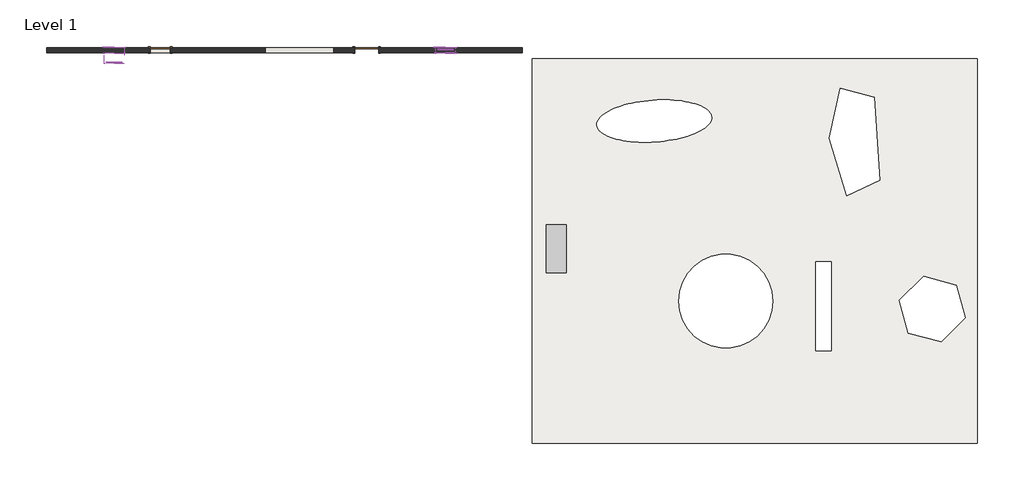
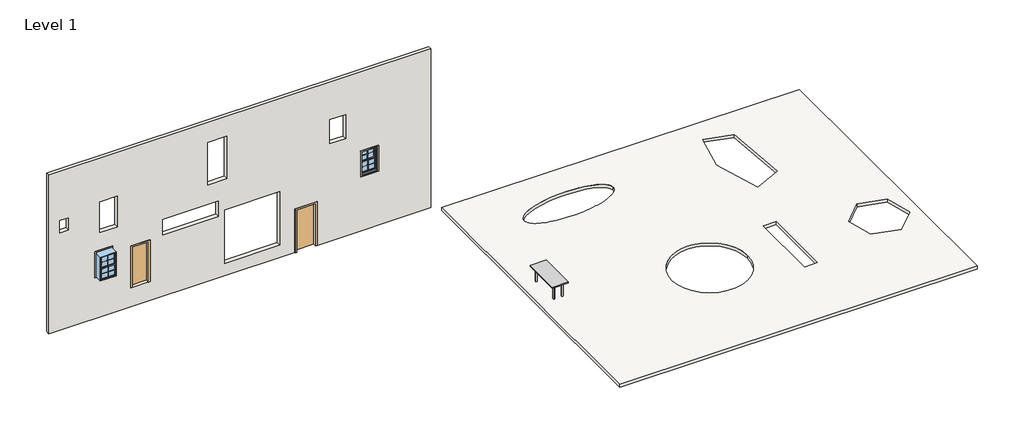
# One storey: 8 proxies, 2 doors, 2 windows, 1 furniture element, 1 slab, 1 wall.
"""IFC4 building model written with IfcOpenShell, lengths in millimetres."""

import ifcopenshell
import ifcopenshell.guid

model = None  # the IFC model being written
_history = None  # IfcOwnerHistory: only IFC2X3 demands one
_inside = {}  # id of a spatial element -> (the spatial element, [elements in it])
_under = {}  # id of a project, library or spatial element -> (it, [spatial elements below it])
_declared = {}  # id of a project -> (the project, [libraries it declares])
_typed = {}  # id of a type object -> (the type object, [elements of that type])
_made_of = {}  # id of a material, layer set ... -> (it, [elements and type objects made of it])


def new_model(schema):
    """Start an empty IFC model of exactly this schema.

    Asked for "IFC4X3", IfcOpenShell would pick the latest addendum, in which some entities
    have other attributes; the version numbers below select the first issue.
    IFC2X3 requires an IfcOwnerHistory on every rooted entity: one is made here for all.
    """
    global model, _history
    if schema == "IFC4X3":
        model = ifcopenshell.file(schema_version=(4, 3, 0, 0))
    else:
        model = ifcopenshell.file(schema=schema)
    _inside.clear()
    _under.clear()
    _declared.clear()
    _typed.clear()
    _made_of.clear()
    _history = None
    if model.schema == "IFC2X3":
        org = make("IfcOrganization", Name="unknown")
        user = make(
            "IfcPersonAndOrganization",
            ThePerson=make("IfcPerson", FamilyName="unknown"),
            TheOrganization=org,
        )
        app = make(
            "IfcApplication",
            ApplicationDeveloper=org,
            Version="unknown",
            ApplicationFullName="unknown",
            ApplicationIdentifier="unknown",
        )
        _history = make(
            "IfcOwnerHistory",
            OwningUser=user,
            OwningApplication=app,
            ChangeAction="ADDED",
            CreationDate=0,
        )
    return model


def make(cls, **values):
    """One entity of the class cls with the attributes given. An attribute that is None is left unset."""
    return model.create_entity(
        cls, **{name: value for name, value in values.items() if value is not None}
    )


def rooted(cls, **values):
    """An entity with a GlobalId (a new one), such as an element, a storey or a relation."""
    return make(cls, GlobalId=ifcopenshell.guid.new(), OwnerHistory=_history, **values)


def si_unit(unit_type, name, prefix=None):
    """IfcSIUnit, for example si_unit("LENGTHUNIT", "METRE", prefix="MILLI")."""
    return make("IfcSIUnit", UnitType=unit_type, Prefix=prefix, Name=name)


def assignment(units):
    """IfcUnitAssignment: the units of a project."""
    return None if units is None else make("IfcUnitAssignment", Units=units)


def point(xyz):
    """IfcCartesianPoint."""
    return None if xyz is None else make("IfcCartesianPoint", Coordinates=xyz)


def direction(xyz):
    """IfcDirection."""
    return None if xyz is None else make("IfcDirection", DirectionRatios=xyz)


def frame(location, z_axis=None, x_axis=None):
    """IfcAxis2Placement3D, a coordinate frame: its origin and axes. An axis left out is left unset."""
    return make(
        "IfcAxis2Placement3D",
        Location=point(location),
        Axis=direction(z_axis),
        RefDirection=direction(x_axis),
    )


def origin():
    """The frame at (0, 0, 0) with its axes left unset."""
    return frame((0.0, 0.0, 0.0))


def origin_with_axes():
    """The frame at (0, 0, 0) with the z axis (0, 0, 1) and the x axis (1, 0, 0) written out."""
    return frame((0.0, 0.0, 0.0), z_axis=(0.0, 0.0, 1.0), x_axis=(1.0, 0.0, 0.0))


def place(relative_to, where):
    """IfcLocalPlacement: puts the frame where relative to a parent placement (None: the world)."""
    return make(
        "IfcLocalPlacement", PlacementRelTo=relative_to, RelativePlacement=where
    )


def context(
    kind, dimensions, precision=None, world=None, true_north=None, identifier=None
):
    """IfcGeometricRepresentationContext, for example the 3D "Model" context."""
    return make(
        "IfcGeometricRepresentationContext",
        ContextIdentifier=identifier,
        ContextType=kind,
        CoordinateSpaceDimension=dimensions,
        Precision=precision,
        WorldCoordinateSystem=world,
        TrueNorth=true_north,
    )


def project(units=None, contexts=None):
    """IfcProject with its units and contexts."""
    return rooted(
        "IfcProject",
        Name="project",
        RepresentationContexts=contexts,
        UnitsInContext=assignment(units),
    )


def spatial(cls, under=None, at=None, **own):
    """A site, building, storey or space (cls), placed at a placement, below another one or the project."""
    s = rooted(cls, ObjectPlacement=at, **own)
    if under is not None:
        _under.setdefault(under.id(), (under, []))[1].append(s)
    return s


def polyline(points):
    """IfcPolyline through the points."""
    return make("IfcPolyline", Points=[point(p) for p in points])


def circle_curve(where, radius):
    """IfcCircle in the frame where."""
    return make("IfcCircle", Position=where, Radius=radius)


def ellipse_curve(where, semi_axis1, semi_axis2):
    """IfcEllipse in the frame where."""
    return make(
        "IfcEllipse", Position=where, SemiAxis1=semi_axis1, SemiAxis2=semi_axis2
    )


def trimmed(basis, trim1, trim2, sense, master):
    """IfcTrimmedCurve: the piece of a basis curve between two trims."""
    return make(
        "IfcTrimmedCurve",
        BasisCurve=basis,
        Trim1=trim1,
        Trim2=trim2,
        SenseAgreement=sense,
        MasterRepresentation=master,
    )


def outline(outer, holes=None, kind="AREA"):
    """IfcArbitraryClosedProfileDef: a profile drawn as a closed curve; with holes, ...WithVoids."""
    if holes is None:
        return make("IfcArbitraryClosedProfileDef", ProfileType=kind, OuterCurve=outer)
    return make(
        "IfcArbitraryProfileDefWithVoids",
        ProfileType=kind,
        OuterCurve=outer,
        InnerCurves=holes,
    )


def extrude(swept, where, along, depth):
    """IfcExtrudedAreaSolid: the profile swept, set in the frame where, extruded along a direction by depth."""
    return make(
        "IfcExtrudedAreaSolid",
        SweptArea=swept,
        Position=where,
        ExtrudedDirection=direction(along),
        Depth=depth,
    )


def shape(context_of_items, identifier, shape_type, items):
    """IfcShapeRepresentation: the items that make up one representation, for example the "Body"."""
    return make(
        "IfcShapeRepresentation",
        ContextOfItems=context_of_items,
        RepresentationIdentifier=identifier,
        RepresentationType=shape_type,
        Items=items,
    )


def source(mapping_origin, context_of_items, identifier, shape_type, items):
    """IfcRepresentationMap: a shape defined once, which mapped items show again and again."""
    return make(
        "IfcRepresentationMap",
        MappingOrigin=mapping_origin,
        MappedRepresentation=shape(context_of_items, identifier, shape_type, items),
    )


def transform(
    local_origin,
    x_axis=None,
    y_axis=None,
    z_axis=None,
    scale=None,
    scale2=None,
    scale3=None,
    uniform=True,
):
    """IfcCartesianTransformationOperator3D, or its non-uniform kind. x_axis, y_axis, z_axis: its Axis1, 2, 3."""
    if uniform:
        return make(
            "IfcCartesianTransformationOperator3D",
            Axis1=direction(x_axis),
            Axis2=direction(y_axis),
            LocalOrigin=point(local_origin),
            Scale=scale,
            Axis3=direction(z_axis),
        )
    return make(
        "IfcCartesianTransformationOperator3DnonUniform",
        Axis1=direction(x_axis),
        Axis2=direction(y_axis),
        LocalOrigin=point(local_origin),
        Scale=scale,
        Axis3=direction(z_axis),
        Scale2=scale2,
        Scale3=scale3,
    )


def mapped(mapping_source, mapping_target):
    """IfcMappedItem: shows the shape of a source again, moved by a transform."""
    return make(
        "IfcMappedItem", MappingSource=mapping_source, MappingTarget=mapping_target
    )


def made_of(thing, what):
    """Note that an element or type object is made of a material, layer set ...; save() writes the relation."""
    if what is not None:
        _made_of.setdefault(what.id(), (what, []))[1].append(thing)
    return thing


def element(
    cls,
    number,
    at=None,
    inside=None,
    cuts=None,
    type_object=None,
    material=None,
    context=None,
    identifier="Body",
    shape_type=None,
    held_by="IfcProductDefinitionShape",
    body=None,
    shapes=None,
    **own,
):
    """One element of the class cls, such as IfcWall. Its Tag is "e" and its number.

    at: its placement. inside: the storey or other place that contains it. cuts: it is an
    opening in that element (IfcRelVoidsElement). A single representation is given by context,
    identifier, shape_type and body (its items); several are given by shapes. held_by: the class
    of the entity that holds the representations. save() writes the other relations.
    """
    e = rooted(cls, Tag="e%d" % number, ObjectPlacement=at, **own)
    if body is not None:
        shapes = [shape(context, identifier, shape_type, body)]
    if shapes is not None:
        e.Representation = make(held_by, Representations=shapes)
    if inside is not None:
        _inside.setdefault(inside.id(), (inside, []))[1].append(e)
    if cuts is not None:
        rooted(
            "IfcRelVoidsElement", RelatingBuildingElement=cuts, RelatedOpeningElement=e
        )
    if type_object is not None:
        _typed.setdefault(type_object.id(), (type_object, []))[1].append(e)
    return made_of(e, material)


def aggregate(whole, parts):
    """IfcRelAggregates: a whole, such as a stair, and the parts it consists of."""
    return rooted("IfcRelAggregates", RelatingObject=whole, RelatedObjects=parts)


def save(model, path):
    """Write the relations noted so far, then the file.

    IfcRelAggregates (storeys below a building ...), IfcRelContainedInSpatialStructure (elements
    in a storey), IfcRelDefinesByType, IfcRelAssociatesMaterial and IfcRelDeclares: one each for
    every whole, place, type object, material and project.
    """
    for whole, parts in _under.values():
        aggregate(whole, parts)
    for where, things in _inside.values():
        rooted(
            "IfcRelContainedInSpatialStructure",
            RelatedElements=things,
            RelatingStructure=where,
        )
    for kind, things in _typed.values():
        rooted("IfcRelDefinesByType", RelatedObjects=things, RelatingType=kind)
    for what, things in _made_of.values():
        rooted("IfcRelAssociatesMaterial", RelatedObjects=things, RelatingMaterial=what)
    for by, libraries in _declared.values():
        rooted("IfcRelDeclares", RelatingContext=by, RelatedDefinitions=libraries)
    model.write(path)


def plane_surface(at):
    """IfcPlane: the flat surface through the origin of the frame at, square to its z axis."""
    return make("IfcPlane", Position=at)


def revolved_surface(curve, axis_point, axis_direction):
    """IfcSurfaceOfRevolution: the curve turned about the line through axis_point along axis_direction."""
    return make(
        "IfcSurfaceOfRevolution",
        SweptCurve=make("IfcArbitraryOpenProfileDef", ProfileType="CURVE", Curve=curve),
        AxisPosition=make("IfcAxis1Placement", Location=point(axis_point), Axis=direction(axis_direction)),
    )


def extruded_surface(curve, direction_of_extrusion, depth):
    """IfcSurfaceOfLinearExtrusion: the curve pushed along a direction by depth."""
    return make(
        "IfcSurfaceOfLinearExtrusion",
        SweptCurve=make("IfcArbitraryOpenProfileDef", ProfileType="CURVE", Curve=curve),
        ExtrudedDirection=direction(direction_of_extrusion),
        Depth=depth,
    )


def advanced_brep(points, edges, surfaces, faces):
    """IfcAdvancedBrep: a solid bounded by faces that lie on surfaces and meet in shared edges.

    An edge is (start, end): straight between two places in points (the first is 0);
    or (start, end, curve); or (start, end, curve, False) where it runs against its curve.
    A face is (place in surfaces, loops), or (place, loops, False) where it looks against
    its surface's normal. A loop lists edges by number (the first is 1), with a minus sign
    where the edge is run from its end to its start. The first loop is the outer one.
    """
    corners = [point(p) for p in points]
    vertices = [make("IfcVertexPoint", VertexGeometry=c) for c in corners]
    made = []
    for start, end, *more in edges:
        made.append(
            make(
                "IfcEdgeCurve",
                EdgeStart=vertices[start],
                EdgeEnd=vertices[end],
                EdgeGeometry=more[0] if more else make("IfcPolyline", Points=[corners[start], corners[end]]),
                SameSense=more[1] if len(more) > 1 else True,
            )
        )
    hull = []
    for where, loops, *sense in faces:
        bounds = []
        for j, loop in enumerate(loops):
            ring = [make("IfcOrientedEdge", EdgeElement=made[abs(k) - 1], Orientation=k > 0) for k in loop]
            bounds.append(
                make(
                    "IfcFaceOuterBound" if j == 0 else "IfcFaceBound",
                    Bound=make("IfcEdgeLoop", EdgeList=ring),
                    Orientation=True,
                )
            )
        hull.append(make("IfcAdvancedFace", Bounds=bounds, FaceSurface=surfaces[where], SameSense=sense[0] if sense else True))
    return make("IfcAdvancedBrep", Outer=make("IfcClosedShell", CfsFaces=hull))


def m_muntin_pattern_2x2_m_muntin_pattern_2x2_aaec3afb(model_context):
    return source(origin(), model_context, "Body", "SweptSolid", [
        extrude(outline(polyline([(257.1375, -6.35), (257.1375, -298.8), (244.4375, -298.8), (244.4375, -6.35), (0.0, -6.35), (0.0, 6.35), (244.4375, 6.35), (244.4375, 298.8), (257.1375, 298.8), (257.1375, 6.35), (501.575, 6.35), (501.575, -6.35), (257.1375, -6.35)])), frame((0.0, 9.525, 0.0), z_axis=(0.0, 1.0, 0.0), x_axis=(0.0, 0.0, 1.0)), (0.0, 0.0, 1.0), 12.7),
        extrude(outline(polyline([(257.1375, -6.35), (257.1375, -298.8), (244.4375, -298.8), (244.4375, -6.35), (0.0, -6.35), (0.0, 6.35), (244.4375, 6.35), (244.4375, 298.8), (257.1375, 298.8), (257.1375, 6.35), (501.575, 6.35), (501.575, -6.35), (257.1375, -6.35)])), frame((0.0, -22.225, 0.0), z_axis=(0.0, 1.0, 0.0), x_axis=(0.0, 0.0, 1.0)), (0.0, 0.0, 1.0), 12.7),
    ])


def m_trim_window_exterior_flat_with_sill_e7ff6350(model_context):
    return source(origin(), model_context, "Body", "SweptSolid", [
        extrude(outline(polyline([(435.0, -1220.4323709), (435.0, -1280.4323709), (-435.0, -1280.4323709), (-435.0, -1220.4323709), (435.0, -1220.4323709)])), origin_with_axes(), (0.0, 0.0, 1.0), 19.05),
        extrude(outline(polyline([(-1230.0, 38.1), (-1202.4580645, 38.1), (-1200.0, 19.05), (-1200.0, 0.0), (-1220.4323709, 0.0), (-1220.4323709, 19.05), (-1230.0, 19.05), (-1230.0, 38.1)])), frame((-447.7, 0.0, 0.0), z_axis=(1.0, 0.0, 0.0), x_axis=(0.0, 1.0, 0.0)), (0.0, 0.0, 1.0), 895.4),
        extrude(outline(polyline([(-435.0, 60.0), (435.0, 60.0), (435.0, -1200.0), (375.0, -1200.0), (375.0, 0.0), (-375.0, 0.0), (-375.0, -1200.0), (-435.0, -1200.0), (-435.0, 60.0)])), origin_with_axes(), (0.0, 0.0, 1.0), 19.05),
    ])


def m_trim_window_interior_flat_picture_frame_31bd2320(model_context):
    return source(origin(), model_context, "Body", "SweptSolid", [
        extrude(outline(polyline([(422.3, 47.3), (422.3, -1247.3), (-422.3, -1247.3), (-422.3, 47.3), (422.3, 47.3)]), holes=[polyline([(362.3, -12.7), (-362.3, -12.7), (-362.3, -1187.3), (362.3, -1187.3), (362.3, -12.7)])]), origin_with_axes(), (0.0, 0.0, 1.0), 30.0),
    ])


def m_single_flush_0762_x_2032mm_0c256fab(model_context):
    return source(origin(), model_context, "Body", "SweptSolid", [
        extrude(outline(polyline([(2108.0, -457.0), (0.0, -457.0), (0.0, -381.0), (2032.0, -381.0), (2032.0, 381.0), (0.0, 381.0), (0.0, 457.0), (2108.0, 457.0), (2108.0, -457.0)])), frame((0.0, 100.0, 0.0), z_axis=(0.0, 1.0, 0.0), x_axis=(0.0, 0.0, 1.0)), (0.0, 0.0, 1.0), 25.0),
        extrude(outline(polyline([(2108.0, 457.0), (2108.0, -457.0), (0.0, -457.0), (0.0, -381.0), (2032.0, -381.0), (2032.0, 381.0), (0.0, 381.0), (0.0, 457.0), (2108.0, 457.0)])), frame((0.0, -125.0, 0.0), z_axis=(0.0, 1.0, 0.0), x_axis=(0.0, 0.0, 1.0)), (0.0, 0.0, 1.0), 25.0),
        extrude(outline(polyline([(381.0, 49.0), (-381.0, 49.0), (-381.0, 100.0), (381.0, 100.0), (381.0, 49.0)])), origin_with_axes(), (0.0, 0.0, 1.0), 2032.0),
    ])


def m_single_flush_0915_x_2134mm_727434cd(model_context):
    return source(origin(), model_context, "Body", "SweptSolid", [
        extrude(outline(polyline([(2210.0, -533.5), (0.0, -533.5), (0.0, -457.5), (2134.0, -457.5), (2134.0, 457.5), (0.0, 457.5), (0.0, 533.5), (2210.0, 533.5), (2210.0, -533.5)])), frame((0.0, -125.0, 0.0), z_axis=(0.0, 1.0, 0.0), x_axis=(0.0, 0.0, 1.0)), (0.0, 0.0, 1.0), 25.0),
        extrude(outline(polyline([(2210.0, 533.5), (2210.0, -533.5), (0.0, -533.5), (0.0, -457.5), (2134.0, -457.5), (2134.0, 457.5), (0.0, 457.5), (0.0, 533.5), (2210.0, 533.5)])), frame((0.0, 100.0, 0.0), z_axis=(0.0, 1.0, 0.0), x_axis=(0.0, 0.0, 1.0)), (0.0, 0.0, 1.0), 25.0),
        extrude(outline(polyline([(457.5, -49.0), (457.5, -100.0), (-457.5, -100.0), (-457.5, -49.0), (457.5, -49.0)])), origin_with_axes(), (0.0, 0.0, 1.0), 2134.0),
    ])


def m_table_rectangular_1830_x_0762mm_a0b3b7a0(model_context):
    return source(origin(), model_context, "Body", "SweptSolid", [
        extrude(outline(polyline([(699.1, 190.5), (699.1, 165.1), (-699.1, 165.1), (-699.1, 190.5), (699.1, 190.5)])), frame((0.0, 0.0, 609.6), z_axis=(0.0, 0.0, 1.0), x_axis=(1.0, 0.0, 0.0)), (0.0, 0.0, 1.0), 101.6),
        extrude(outline(polyline([(699.1, -190.5), (-699.1, -190.5), (-699.1, -165.1), (699.1, -165.1), (699.1, -190.5)])), frame((0.0, 0.0, 609.6), z_axis=(0.0, 0.0, 1.0), x_axis=(1.0, 0.0, 0.0)), (0.0, 0.0, 1.0), 101.6),
        extrude(outline(polyline([(-711.8, -165.1), (-737.2, -165.1), (-737.2, 165.1), (-711.8, 165.1), (-711.8, -165.1)])), frame((0.0, 0.0, 609.6), z_axis=(0.0, 0.0, 1.0), x_axis=(1.0, 0.0, 0.0)), (0.0, 0.0, 1.0), 101.6),
        extrude(outline(polyline([(711.8, -165.1), (711.8, 165.1), (737.2, 165.1), (737.2, -165.1), (711.8, -165.1)])), frame((0.0, 0.0, 609.6), z_axis=(0.0, 0.0, 1.0), x_axis=(1.0, 0.0, 0.0)), (0.0, 0.0, 1.0), 101.6),
        extrude(outline(polyline([(915.0, 381.0), (915.0, -381.0), (-915.0, -381.0), (-915.0, 381.0), (915.0, 381.0)])), frame((0.0, 0.0, 711.2), z_axis=(0.0, 0.0, 1.0), x_axis=(1.0, 0.0, 0.0)), (0.0, 0.0, 1.0), 50.8),
        extrude(outline(polyline([(-699.1, 228.6), (-699.1, 165.1), (-762.6, 165.1), (-762.6, 228.6), (-699.1, 228.6)])), origin_with_axes(), (0.0, 0.0, 1.0), 711.2),
        extrude(outline(polyline([(699.1, 228.6), (762.6, 228.6), (762.6, 165.1), (699.1, 165.1), (699.1, 228.6)])), origin_with_axes(), (0.0, 0.0, 1.0), 711.2),
        extrude(outline(polyline([(-699.1, -228.6), (-762.6, -228.6), (-762.6, -165.1), (-699.1, -165.1), (-699.1, -228.6)])), origin_with_axes(), (0.0, 0.0, 1.0), 711.2),
        extrude(outline(polyline([(699.1, -228.6), (699.1, -165.1), (762.6, -165.1), (762.6, -228.6), (699.1, -228.6)])), origin_with_axes(), (0.0, 0.0, 1.0), 711.2),
    ])


def m_window_double_hung_750_x_1200mm_e21ea802(model_context):
    return source(origin(), model_context, "Body", "SweptSolid", [
        extrude(outline(polyline([(298.8, -469.85), (298.8, -476.2), (-298.8, -476.2), (-298.8, -469.85), (298.8, -469.85)])), frame((0.0, 0.0, 990.6), z_axis=(0.0, 0.0, 1.0), x_axis=(1.0, 0.0, 0.0)), (0.0, 0.0, 1.0), 501.575),
        extrude(outline(polyline([(-298.8, -482.55), (298.8, -482.55), (298.8, -488.9), (-298.8, -488.9), (-298.8, -482.55)])), frame((0.0, 0.0, 990.6), z_axis=(0.0, 0.0, 1.0), x_axis=(1.0, 0.0, 0.0)), (0.0, 0.0, 1.0), 501.575),
        extrude(outline(polyline([(298.8, -425.4), (298.8, -431.75), (-298.8, -431.75), (-298.8, -425.4), (298.8, -425.4)])), frame((0.0, 0.0, 1536.625), z_axis=(0.0, 0.0, 1.0), x_axis=(1.0, 0.0, 0.0)), (0.0, 0.0, 1.0), 501.575),
        extrude(outline(polyline([(-298.8, -438.1), (298.8, -438.1), (298.8, -444.45), (-298.8, -444.45), (-298.8, -438.1)])), frame((0.0, 0.0, 1536.625), z_axis=(0.0, 0.0, 1.0), x_axis=(1.0, 0.0, 0.0)), (0.0, 0.0, 1.0), 501.575),
        extrude(outline(polyline([(1536.625, -343.25), (946.15, -343.25), (946.15, 343.25), (1536.625, 343.25), (1536.625, -343.25)]), holes=[polyline([(1492.175, 298.8), (990.6, 298.8), (990.6, -298.8), (1492.175, -298.8), (1492.175, 298.8)])]), frame((0.0, -501.6, 0.0), z_axis=(0.0, 1.0, 0.0), x_axis=(0.0, 0.0, 1.0)), (0.0, 0.0, 1.0), 44.45),
        extrude(outline(polyline([(2082.65, -343.25), (1492.175, -343.25), (1492.175, 343.25), (2082.65, 343.25), (2082.65, -343.25)]), holes=[polyline([(2038.2, 298.8), (1536.625, 298.8), (1536.625, -298.8), (2038.2, -298.8), (2038.2, 298.8)])]), frame((0.0, -457.15, 0.0), z_axis=(0.0, 1.0, 0.0), x_axis=(0.0, 0.0, 1.0)), (0.0, 0.0, 1.0), 44.45),
        extrude(outline(polyline([(2114.4, -375.0), (914.4, -375.0), (914.4, 375.0), (2114.4, 375.0), (2114.4, -375.0)]), holes=[polyline([(2082.65, 343.25), (946.15, 343.25), (946.15, -343.25), (2082.65, -343.25), (2082.65, 343.25)])]), frame((0.0, -514.3, 0.0), z_axis=(0.0, 1.0, 0.0), x_axis=(0.0, 0.0, 1.0)), (0.0, 0.0, 1.0), 633.35),
    ])


def m_window_double_hung_750_x_1200mm_41070976(model_context):
    return source(origin(), model_context, "Body", "SweptSolid", [
        extrude(outline(polyline([(298.8, 30.15), (298.8, 23.8), (-298.8, 23.8), (-298.8, 30.15), (298.8, 30.15)])), frame((0.0, 0.0, 990.6), z_axis=(0.0, 0.0, 1.0), x_axis=(1.0, 0.0, 0.0)), (0.0, 0.0, 1.0), 501.575),
        extrude(outline(polyline([(-298.8, 17.45), (298.8, 17.45), (298.8, 11.1), (-298.8, 11.1), (-298.8, 17.45)])), frame((0.0, 0.0, 990.6), z_axis=(0.0, 0.0, 1.0), x_axis=(1.0, 0.0, 0.0)), (0.0, 0.0, 1.0), 501.575),
        extrude(outline(polyline([(298.8, 74.6), (298.8, 68.25), (-298.8, 68.25), (-298.8, 74.6), (298.8, 74.6)])), frame((0.0, 0.0, 1536.625), z_axis=(0.0, 0.0, 1.0), x_axis=(1.0, 0.0, 0.0)), (0.0, 0.0, 1.0), 501.575),
        extrude(outline(polyline([(-298.8, 61.9), (298.8, 61.9), (298.8, 55.55), (-298.8, 55.55), (-298.8, 61.9)])), frame((0.0, 0.0, 1536.625), z_axis=(0.0, 0.0, 1.0), x_axis=(1.0, 0.0, 0.0)), (0.0, 0.0, 1.0), 501.575),
        extrude(outline(polyline([(1536.625, -343.25), (946.15, -343.25), (946.15, 343.25), (1536.625, 343.25), (1536.625, -343.25)]), holes=[polyline([(1492.175, 298.8), (990.6, 298.8), (990.6, -298.8), (1492.175, -298.8), (1492.175, 298.8)])]), frame((0.0, -1.6, 0.0), z_axis=(0.0, 1.0, 0.0), x_axis=(0.0, 0.0, 1.0)), (0.0, 0.0, 1.0), 44.45),
        extrude(outline(polyline([(2082.65, -343.25), (1492.175, -343.25), (1492.175, 343.25), (2082.65, 343.25), (2082.65, -343.25)]), holes=[polyline([(2038.2, 298.8), (1536.625, 298.8), (1536.625, -298.8), (2038.2, -298.8), (2038.2, 298.8)])]), frame((0.0, 42.85, 0.0), z_axis=(0.0, 1.0, 0.0), x_axis=(0.0, 0.0, 1.0)), (0.0, 0.0, 1.0), 44.45),
        extrude(outline(polyline([(2114.4, -375.0), (914.4, -375.0), (914.4, 375.0), (2114.4, 375.0), (2114.4, -375.0)]), holes=[polyline([(2082.65, 343.25), (946.15, 343.25), (946.15, -343.25), (2082.65, -343.25), (2082.65, 343.25)])]), frame((0.0, -14.3, 0.0), z_axis=(0.0, 1.0, 0.0), x_axis=(0.0, 0.0, 1.0)), (0.0, 0.0, 1.0), 133.35),
        extrude(outline(polyline([(2114.4, 375.0), (2114.4, -375.0), (914.4, -375.0), (914.4, 375.0), (2114.4, 375.0)]), holes=[polyline([(2095.35, 355.95), (933.45, 355.95), (933.45, -355.95), (2095.35, -355.95), (2095.35, 355.95)])]), frame((0.0, -100.0, 0.0), z_axis=(0.0, 1.0, 0.0), x_axis=(0.0, 0.0, 1.0)), (0.0, 0.0, 1.0), 85.7),
    ])


model = new_model("IFC4")

# Units and contexts
model_context = context("Model", 3, world=origin())
ifc_project = project(units=[si_unit("LENGTHUNIT", "METRE", prefix="MILLI")], contexts=[model_context])

# Site, building, storey
site = spatial("IfcSite", under=ifc_project)
building = spatial("IfcBuilding", under=site)
storey = spatial("IfcBuildingStorey", under=building, Name="Level 1", Elevation=0.0)

# Proxies
placement = place(None, origin())
m_muntin_pattern_2x2_m_muntin_pattern_2x2_shape = m_muntin_pattern_2x2_m_muntin_pattern_2x2_aaec3afb(model_context)
element("IfcBuildingElementProxy", 1, Name="M_Muntin Pattern_2x2 : M_Muntin Pattern_2x2", ObjectType="M_Muntin Pattern_2x2 : M_Muntin Pattern_2x2", at=placement, inside=storey, context=model_context, shape_type="MappedRepresentation", body=[
    mapped(m_muntin_pattern_2x2_m_muntin_pattern_2x2_shape, transform((-13755.2543844, 2099.5505832, 3404.9440493), x_axis=(1.0, 0.0, 0.0), y_axis=(0.0, 1.0, 0.0), z_axis=(0.0, 0.0, 1.0))),
])
element("IfcBuildingElementProxy", 2, Name="M_Muntin Pattern_2x2 : M_Muntin Pattern_2x2", ObjectType="M_Muntin Pattern_2x2 : M_Muntin Pattern_2x2", at=placement, inside=storey, context=model_context, shape_type="MappedRepresentation", body=[
    mapped(m_muntin_pattern_2x2_m_muntin_pattern_2x2_shape, transform((-13755.2543844, 2055.1005832, 2858.9190493), x_axis=(1.0, 0.0, 0.0), y_axis=(0.0, 1.0, 0.0), z_axis=(0.0, 0.0, 1.0))),
])
element("IfcBuildingElementProxy", 3, Name="M_Muntin Pattern_2x2 : M_Muntin Pattern_2x2", ObjectType="M_Muntin Pattern_2x2 : M_Muntin Pattern_2x2", at=placement, inside=storey, context=model_context, shape_type="MappedRepresentation", body=[
    mapped(m_muntin_pattern_2x2_m_muntin_pattern_2x2_shape, transform((-26427.6862127, 1599.5505832, 2762.3712435), x_axis=(1.0, 0.0, 0.0), y_axis=(0.0, 1.0, 0.0), z_axis=(0.0, 0.0, 1.0))),
])
element("IfcBuildingElementProxy", 4, Name="M_Muntin Pattern_2x2 : M_Muntin Pattern_2x2", ObjectType="M_Muntin Pattern_2x2 : M_Muntin Pattern_2x2", at=placement, inside=storey, context=model_context, shape_type="MappedRepresentation", body=[
    mapped(m_muntin_pattern_2x2_m_muntin_pattern_2x2_shape, transform((-26427.6862127, 1555.1005832, 2216.3462435), x_axis=(1.0, 0.0, 0.0), y_axis=(0.0, 1.0, 0.0), z_axis=(0.0, 0.0, 1.0))),
])
m_trim_window_exterior_flat_with_sill_shape = m_trim_window_exterior_flat_with_sill_e7ff6350(model_context)
element("IfcBuildingElementProxy", 5, Name="M_Trim-Window-Exterior-Flat : with Sill", ObjectType="M_Trim-Window-Exterior-Flat : with Sill", at=placement, inside=storey, context=model_context, shape_type="MappedRepresentation", body=[
    mapped(m_trim_window_exterior_flat_with_sill_shape, transform((-13755.2543844, 2134.4755832, 3982.7190493), x_axis=(-1.0, 0.0, 0.0), y_axis=(0.0, 0.0, 1.0), z_axis=(0.0, 1.0, 0.0))),
])
element("IfcBuildingElementProxy", 6, Name="M_Trim-Window-Exterior-Flat : with Sill", ObjectType="M_Trim-Window-Exterior-Flat : with Sill", at=placement, inside=storey, context=model_context, shape_type="MappedRepresentation", body=[
    mapped(m_trim_window_exterior_flat_with_sill_shape, transform((-26427.6862127, 2134.4755832, 3340.1462435), x_axis=(-1.0, 0.0, 0.0), y_axis=(0.0, 0.0, 1.0), z_axis=(0.0, 1.0, 0.0))),
])
m_trim_window_interior_flat_picture_frame_shape = m_trim_window_interior_flat_picture_frame_31bd2320(model_context)
element("IfcBuildingElementProxy", 7, Name="M_Trim-Window-Interior-Flat : Picture Frame", ObjectType="M_Trim-Window-Interior-Flat : Picture Frame", at=placement, inside=storey, context=model_context, shape_type="MappedRepresentation", body=[
    mapped(m_trim_window_interior_flat_picture_frame_shape, transform((-13755.2543844, 1934.4755832, 3982.7190493), x_axis=(1.0, 0.0, 0.0), y_axis=(0.0, 0.0, 1.0), z_axis=(0.0, -1.0, 0.0))),
])
element("IfcBuildingElementProxy", 8, Name="M_Trim-Window-Interior-Flat : Picture Frame", ObjectType="M_Trim-Window-Interior-Flat : Picture Frame", at=placement, inside=storey, context=model_context, shape_type="MappedRepresentation", body=[
    mapped(m_trim_window_interior_flat_picture_frame_shape, transform((-26427.6862127, 1934.4755832, 3340.1462435), x_axis=(1.0, 0.0, 0.0), y_axis=(0.0, 0.0, 1.0), z_axis=(0.0, -1.0, 0.0))),
])

# Doors
m_single_flush_0762_x_2032mm_shape = m_single_flush_0762_x_2032mm_0c256fab(model_context)
element("IfcDoor", 9, ObjectType="M_Single-Flush : 0762 x 2032mm", at=placement, inside=storey, context=model_context, shape_type="MappedRepresentation", body=[
    mapped(m_single_flush_0762_x_2032mm_shape, transform((-24671.6862127, 2034.4755832, 968.0), x_axis=(1.0, 0.0, 0.0), y_axis=(0.0, 1.0, 0.0), z_axis=(0.0, 0.0, 1.0))),
])
m_single_flush_0915_x_2134mm_shape = m_single_flush_0915_x_2134mm_727434cd(model_context)
element("IfcDoor", 10, ObjectType="M_Single-Flush : 0915 x 2134mm", at=placement, inside=storey, context=model_context, shape_type="MappedRepresentation", body=[
    mapped(m_single_flush_0915_x_2134mm_shape, transform((-16774.8897659, 2034.4755832, 0.0), x_axis=(-1.0, 0.0, 0.0), y_axis=(0.0, -1.0, 0.0), z_axis=(0.0, 0.0, 1.0))),
])

# Furniture
m_table_rectangular_1830_x_0762mm_shape = m_table_rectangular_1830_x_0762mm_a0b3b7a0(model_context)
element("IfcFurniture", 11, ObjectType="M_Table-Rectangular : 1830 x 0762mm", at=placement, inside=storey, context=model_context, shape_type="MappedRepresentation", body=[
    mapped(m_table_rectangular_1830_x_0762mm_shape, transform((-9517.3897659, -5565.5244168, 0.0), x_axis=(0.0, 1.0, 0.0), y_axis=(-1.0, 0.0, 0.0), z_axis=(0.0, 0.0, 1.0))),
])

# Slab
element("IfcSlab", 12, ObjectType="Generic 150mm", at=placement, inside=storey, context=model_context, shape_type="AdvancedBrep", body=[
    advanced_brep(
    [(-10438.0920872, 1704.9536342, -150.0), (6597.1361468, 1704.9536342, -150.0), (6597.1361468, -12995.0463658, -150.0), (-10438.0920872, -12995.0463658, -150.0), (402.6850474, -6063.7932352, -150.0), (402.6850474, -9463.7932352, -150.0), (1002.6850474, -9463.7932352, -150.0), (1002.6850474, -6063.7932352, -150.0), (-1226.5132944, -7566.8871411, -150.0), (-4826.5132944, -7566.8871411, -150.0), (3950.2905395, -8793.2666419, -150.0), (5205.9941136, -9129.7314005, -150.0), (6125.2329292, -8210.492585, -150.0), (5788.7681706, -6954.7890108, -150.0), (4533.0645964, -6618.3242522, -150.0), (3613.8257808, -7537.5630677, -150.0), (2640.3105602, 236.4658339, -150.0), (1342.8691088, 584.1142231, -150.0), (924.6812259, -1326.1660948, -150.0), (1597.1361468, -3525.6670335, -150.0), (2862.1361468, -2935.7878459, -150.0), (-3571.6563241, -523.7317463, -150.0), (-7960.9381452, -830.6602307, -150.0), (6597.1361468, 1704.9536342, 0.0), (-10438.0920872, 1704.9536342, 0.0), (-10438.0920872, -12995.0463658, 0.0), (6597.1361468, -12995.0463658, 0.0), (402.6850474, -9463.7932352, 0.0), (402.6850474, -6063.7932352, 0.0), (1002.6850474, -6063.7932352, 0.0), (1002.6850474, -9463.7932352, 0.0), (-4826.5132944, -7566.8871411, 0.0), (-1226.5132944, -7566.8871411, 0.0), (5205.9941136, -9129.7314005, 0.0), (3950.2905395, -8793.2666419, 0.0), (3613.8257808, -7537.5630677, 0.0), (4533.0645964, -6618.3242522, 0.0), (5788.7681706, -6954.7890108, 0.0), (6125.2329292, -8210.492585, 0.0), (1342.8691088, 584.1142231, 0.0), (2640.3105602, 236.4658339, 0.0), (2862.1361468, -2935.7878459, 0.0), (1597.1361468, -3525.6670335, 0.0), (924.6812259, -1326.1660948, 0.0), (-7960.9381452, -830.6602307, 0.0), (-3571.6563241, -523.7317463, 0.0)],
    [
        (0, 1),
        (1, 2),
        (2, 3),
        (3, 0),
        (4, 5),
        (5, 6),
        (6, 7),
        (7, 4),
        (8, 9, circle_curve(frame((-3026.5132944, -7566.8871411, -150.0), z_axis=(0.0, 0.0, 1.0), x_axis=(-1.0, 0.0, 0.0)), 1800.0)),
        (9, 8, circle_curve(frame((-3026.5132944, -7566.8871411, -150.0), z_axis=(0.0, 0.0, 1.0), x_axis=(-1.0, 0.0, 0.0)), 1800.0)),
        (10, 11),
        (11, 12),
        (12, 13),
        (13, 14),
        (14, 15),
        (15, 10),
        (16, 17),
        (17, 18),
        (18, 19),
        (19, 20),
        (20, 16),
        (21, 22, ellipse_curve(frame((-5766.2972347, -677.1959885, -150.0), z_axis=(0.0, 0.0, 1.0), x_axis=(-0.9975640502598249, -0.06975647374411696, 0.0)), 2200.0, 800.0)),
        (22, 21, ellipse_curve(frame((-5766.2972347, -677.1959885, -150.0), z_axis=(0.0, 0.0, 1.0), x_axis=(-0.9975640502598249, -0.06975647374411696, 0.0)), 2200.0, 800.0)),
        (23, 24),
        (24, 25),
        (25, 26),
        (26, 23),
        (27, 28),
        (28, 29),
        (29, 30),
        (30, 27),
        (31, 32, circle_curve(frame((-3026.5132944, -7566.8871411, 0.0), z_axis=(0.0, 0.0, -1.0), x_axis=(-1.0, 0.0, 0.0)), 1800.0)),
        (32, 31, circle_curve(frame((-3026.5132944, -7566.8871411, 0.0), z_axis=(0.0, 0.0, -1.0), x_axis=(-1.0, 0.0, 0.0)), 1800.0)),
        (33, 34),
        (34, 35),
        (35, 36),
        (36, 37),
        (37, 38),
        (38, 33),
        (39, 40),
        (40, 41),
        (41, 42),
        (42, 43),
        (43, 39),
        (44, 45, ellipse_curve(frame((-5766.2972347, -677.1959885, 0.0), z_axis=(0.0, 0.0, -1.0), x_axis=(-0.9975640502598249, -0.06975647374411696, 0.0)), 2200.0, 800.0)),
        (45, 44, ellipse_curve(frame((-5766.2972347, -677.1959885, 0.0), z_axis=(0.0, 0.0, -1.0), x_axis=(-0.9975640502598249, -0.06975647374411696, 0.0)), 2200.0, 800.0)),
        (0, 24),
        (23, 1),
        (26, 2),
        (25, 3),
        (4, 28),
        (27, 5),
        (30, 6),
        (29, 7),
        (8, 32),
        (31, 9),
        (10, 34),
        (33, 11),
        (38, 12),
        (37, 13),
        (36, 14),
        (35, 15),
        (16, 40),
        (39, 17),
        (18, 43),
        (42, 19),
        (41, 20),
        (21, 45),
        (44, 22),
    ],
    [
        plane_surface(frame((5561.9079128, 1704.9536342, -150.0), z_axis=(0.0, 0.0, -1.0), x_axis=(1.0, 0.0, 0.0))),
        plane_surface(frame((5561.9079128, 1704.9536342, 0.0), z_axis=(0.0, 0.0, 1.0), x_axis=(-1.0, 0.0, 0.0))),
        plane_surface(frame((-10438.0920872, 1704.9536342, -150.0), z_axis=(0.0, 1.0, 0.0), x_axis=(0.0, 0.0, 1.0))),
        plane_surface(frame((6597.1361468, 1704.9536342, -150.0), z_axis=(1.0, 0.0, 0.0), x_axis=(0.0, 0.0, 1.0))),
        plane_surface(frame((6597.1361468, -12995.0463658, -150.0), z_axis=(0.0, -1.0, 0.0), x_axis=(0.0, 0.0, 1.0))),
        plane_surface(frame((-10438.0920872, -12995.0463658, -150.0), z_axis=(-1.0, 0.0, 0.0), x_axis=(0.0, 0.0, 1.0))),
        plane_surface(frame((402.6850474, -6063.7932352, 754.8), z_axis=(1.0, 0.0, 0.0), x_axis=(0.0, 0.0, -1.0))),
        plane_surface(frame((402.6850474, -9463.7932352, 754.8), z_axis=(0.0, 1.0, 0.0), x_axis=(0.0, 0.0, -1.0))),
        plane_surface(frame((1002.6850474, -9463.7932352, 754.8), z_axis=(-1.0, 0.0, 0.0), x_axis=(0.0, 0.0, -1.0))),
        plane_surface(frame((1002.6850474, -6063.7932352, 754.8), z_axis=(0.0, -1.0, 0.0), x_axis=(0.0, 0.0, -1.0))),
        revolved_surface(polyline([(-4826.5132944, -7566.8871411, 0.0), (-4826.5132944, -7566.8871411, -150.0)]), (-3026.5132944, -7566.8871411, -454.8), (0.0, 0.0, 1.0)),
        plane_surface(frame((3950.2905395, -8793.2666419, 754.8), z_axis=(0.2588190451025399, 0.9659258262890632, 0.0), x_axis=(0.0, 0.0, -1.0))),
        plane_surface(frame((5205.9941136, -9129.7314005, 754.8), z_axis=(-0.7071067811865333, 0.7071067811865619, 0.0), x_axis=(0.0, 0.0, -1.0))),
        plane_surface(frame((6125.2329292, -8210.492585, 754.8), z_axis=(-0.9659258262890744, -0.2588190451024985, 0.0), x_axis=(0.0, 0.0, -1.0))),
        plane_surface(frame((5788.7681706, -6954.7890108, 754.8), z_axis=(-0.25881904510254333, -0.9659258262890623, 0.0), x_axis=(0.0, 0.0, -1.0))),
        plane_surface(frame((4533.0645964, -6618.3242522, 754.8), z_axis=(0.7071067811865306, -0.7071067811865644, 0.0), x_axis=(0.0, 0.0, -1.0))),
        plane_surface(frame((3613.8257808, -7537.5630677, 754.8), z_axis=(0.965925826289073, 0.2588190451025034, 0.0), x_axis=(0.0, 0.0, -1.0))),
        plane_surface(frame((2640.3105602, 236.4658339, -150.0), z_axis=(-0.25881904510253306, -0.9659258262890651, 0.0), x_axis=(0.0, 0.0, 1.0))),
        plane_surface(frame((924.6812259, -1326.1660948, -150.0), z_axis=(0.9563047559630387, 0.29237170472272644, 0.0), x_axis=(0.0, 0.0, 1.0))),
        plane_surface(frame((1597.1361468, -3525.6670335, -150.0), z_axis=(-0.42261826174069067, 0.9063077870366542, 0.0), x_axis=(0.0, 0.0, 1.0))),
        plane_surface(frame((2862.1361468, -2935.7878459, -150.0), z_axis=(-0.997564050259825, -0.06975647374411523, 0.0), x_axis=(0.0, 0.0, 1.0))),
        plane_surface(frame((1342.8691088, 584.1142231, -150.0), z_axis=(0.9768664776736946, -0.21385014565669358, 0.0), x_axis=(0.0, 0.0, 1.0))),
        extruded_surface(trimmed(ellipse_curve(frame((-5766.2972347, -677.1959885, 150.0), z_axis=(0.0, 0.0, 1.0), x_axis=(-0.9975640502598249, -0.06975647374411696, 0.0)), 2200.0, 800.0), [point((-3571.6563241, -523.7317463, 150.0))], [point((-7960.9381452, -830.6602307, 150.0))], True, "CARTESIAN"), (0.0, 0.0, -150.0), 150.0),
        extruded_surface(trimmed(ellipse_curve(frame((-5766.2972347, -677.1959885, 150.0), z_axis=(0.0, 0.0, 1.0), x_axis=(-0.9975640502598249, -0.06975647374411696, 0.0)), 2200.0, 800.0), [point((-7960.9381452, -830.6602307, 150.0))], [point((-3571.6563241, -523.7317463, 150.0))], True, "CARTESIAN"), (0.0, 0.0, -150.0), 150.0),
    ],
    [
        (0, [[1, 2, 3, 4], [5, 6, 7, 8], [9, 10], [11, 12, 13, 14, 15, 16], [17, 18, 19, 20, 21], [22, 23]]),
        (1, [[24, 25, 26, 27], [28, 29, 30, 31], [32, 33], [34, 35, 36, 37, 38, 39], [40, 41, 42, 43, 44], [45, 46]]),
        (2, [[-1, 47, -24, 48]]),
        (3, [[-2, -48, -27, 49]]),
        (4, [[-3, -49, -26, 50]]),
        (5, [[-4, -50, -25, -47]]),
        (6, [[51, -28, 52, -5]]),
        (7, [[-52, -31, 53, -6]]),
        (8, [[-53, -30, 54, -7]]),
        (9, [[-51, -8, -54, -29]]),
        (10, [[55, -32, 56, -9]]),
        (10, [[-55, -10, -56, -33]]),
        (11, [[57, -34, 58, -11]]),
        (12, [[-58, -39, 59, -12]]),
        (13, [[-59, -38, 60, -13]]),
        (14, [[-60, -37, 61, -14]]),
        (15, [[-61, -36, 62, -15]]),
        (16, [[-57, -16, -62, -35]]),
        (17, [[-17, 63, -40, 64]]),
        (18, [[-19, 65, -43, 66]]),
        (19, [[-20, -66, -42, 67]]),
        (20, [[-21, -67, -41, -63]]),
        (21, [[-18, -64, -44, -65]]),
        (22, [[-22, 68, -45, 69]]),
        (23, [[-23, -69, -46, -68]]),
    ],
),
])

# Wall
element("IfcWall", 13, ObjectType="Generic - 200mm", at=placement, inside=storey, context=model_context, shape_type="SweptSolid", body=[
    extrude(outline(polyline([(8000.0, -29017.3897659), (0.0, -29017.3897659), (0.0, -17232.3897659), (2134.0, -17232.3897659), (2134.0, -16317.3897659), (0.0, -16317.3897659), (0.0, -10817.3897659), (8000.0, -10817.3897659), (8000.0, -29017.3897659)]), holes=[polyline([(968.0, -25052.6862127), (3000.0, -25052.6862127), (3000.0, -24290.6862127), (968.0, -24290.6862127), (968.0, -25052.6862127)]), polyline([(4915.0, -28496.5284847), (5525.0, -28496.5284847), (5525.0, -28090.5284847), (4915.0, -28090.5284847), (4915.0, -28496.5284847)]), polyline([(2140.1462435, -26802.6862127), (3340.1462435, -26802.6862127), (3340.1462435, -26052.6862127), (2140.1462435, -26052.6862127), (2140.1462435, -26802.6862127)]), polyline([(2782.7190493, -14130.2543844), (3982.7190493, -14130.2543844), (3982.7190493, -13380.2543844), (2782.7190493, -13380.2543844), (2782.7190493, -14130.2543844)]), polyline([(4914.4, -15639.9853759), (6114.4, -15639.9853759), (6114.4, -14889.9853759), (4914.4, -14889.9853759), (4914.4, -15639.9853759)]), polyline([(4866.0, -20539.9853759), (4866.0, -21454.9853759), (7000.0, -21454.9853759), (7000.0, -20539.9853759), (4866.0, -20539.9853759)]), polyline([(3328.9271244, -20644.8897659), (3328.9271244, -18024.3599995), (634.0, -18024.3599995), (634.0, -20644.8897659), (3328.9271244, -20644.8897659)]), polyline([(3873.453269, -23605.3752389), (3873.453269, -20944.8897659), (3100.0, -20944.8897659), (3100.0, -23605.3752389), (3873.453269, -23605.3752389)]), polyline([(5800.0, -26593.5284847), (5800.0, -25757.3810809), (4260.1064286, -25757.3810809), (4260.1064286, -26593.5284847), (5800.0, -26593.5284847)])]), frame((0.0, 1934.4755832, 0.0), z_axis=(0.0, 1.0, 0.0), x_axis=(0.0, 0.0, 1.0)), (0.0, 0.0, 1.0), 200.0),
])

# Windows
m_window_double_hung_750_x_1200mm_shape = m_window_double_hung_750_x_1200mm_e21ea802(model_context)
element("IfcWindow", 14, ObjectType="M_Window-Double-Hung : 750 x 1200mm", at=placement, inside=storey, context=model_context, shape_type="MappedRepresentation", body=[
    mapped(m_window_double_hung_750_x_1200mm_shape, transform((-26427.6862127, 2034.4755832, 1225.7462435), x_axis=(1.0, 0.0, 0.0), y_axis=(0.0, 1.0, 0.0), z_axis=(0.0, 0.0, 1.0))),
])
m_window_double_hung_750_x_1200mm_2_shape = m_window_double_hung_750_x_1200mm_41070976(model_context)
element("IfcWindow", 15, ObjectType="M_Window-Double-Hung : 750 x 1200mm", at=placement, inside=storey, context=model_context, shape_type="MappedRepresentation", body=[
    mapped(m_window_double_hung_750_x_1200mm_2_shape, transform((-13755.2543844, 2034.4755832, 1868.3190493), x_axis=(1.0, 0.0, 0.0), y_axis=(0.0, 1.0, 0.0), z_axis=(0.0, 0.0, 1.0))),
])

save(model, "model.ifc")

# Revit data of these elements
# Project information
#   Project Issue Date = "Issue Date"
#   Project Status = "Project Status"
#   Client Name = "Owner"
#   Project Address = "Enter address here"
#   Project Name = "Project Name"
#   Project Number = "0001"
# Type "M_Muntin Pattern_2x2 : M_Muntin Pattern_2x2"
#   Width [instance default] = 1200 mm
#   Thickness = 12.7 mm
#   Height [instance default] = 1200 mm
#   Distance = 19.05 mm
#   Interior Material [instance default] = none
#   Exterior Material [instance default] = none
#   Default Elevation = 0
# Type "M_Trim-Window-Exterior-Flat : with Sill"
#   Trim Width = 60 mm
#   Trim Thickness_Picture Frame = 30 mm
#   Trim Thickness_with Sill = 19.05 mm
#   Sill Thickness = 30 mm
#   Opening Width [instance default] = 600 mm
#   Opening Height [instance default] = 900 mm
#   Default Elevation = 1200 mm
#   Sill = yes
#   Picture Frame = no
#   Trim Material [instance default] = none
# Type "M_Trim-Window-Interior-Flat : Picture Frame"
#   Trim Thickness_Picture Frame = 30 mm
#   Trim Width = 60 mm
#   Trim Thickness_with Sill = 20 mm
#   Sill Thickness = 30 mm
#   Opening Width [instance default] = 600 mm
#   Opening Height [instance default] = 900 mm
#   Default Elevation = 1200 mm
#   Sill = no
#   Picture Frame = yes
#   Trim Material [instance default] = none
# Type "M_Single-Flush : 0762 x 2032mm"
#   Type Mark = "28"
#   Construction Type Id = "MDOOR"
#   Analytic Construction = "Metal"
#   Thickness = 51 mm
#   Thermal Resistance (R) = 0.270117 (m²·K)/W
#   Heat Transfer Coefficient (U) = 3.7021 W/(m²·K)
#   Height = 2032 mm
#   Trim Projection Ext = 25 mm
#   Trim Projection Int = 25 mm
#   Trim Width = 76 mm
#   Width = 762 mm
#   Define Thermal Properties by = 1
#   Define Thermal Properties by = 1
#   Door Material = Door - Panel
#   Frame Material = Door - Frame
#   Visual Light Transmittance = 0
#   Solar Heat Gain Coefficient = 0
#   Function = (empty or 0)
#   Wall Closure = (empty or 0)
# Type "M_Single-Flush : 0915 x 2134mm"
#   Type Mark = "20"
#   Construction Type Id = "MDOOR"
#   Analytic Construction = "Metal"
#   Thickness = 51 mm
#   Thermal Resistance (R) = 0.270117 (m²·K)/W
#   Heat Transfer Coefficient (U) = 3.7021 W/(m²·K)
#   Height = 2134 mm
#   Trim Projection Ext = 25 mm
#   Trim Projection Int = 25 mm
#   Trim Width = 76 mm
#   Width = 915 mm
#   Define Thermal Properties by = 1
#   Define Thermal Properties by = 1
#   Door Material = Door - Panel
#   Frame Material = Door - Frame
#   Visual Light Transmittance = 0
#   Solar Heat Gain Coefficient = 0
#   Function = (empty or 0)
#   Wall Closure = (empty or 0)
# Type "M_Table-Rectangular : 1830 x 0762mm"
#   Height = 762 mm
#   Length = 1830 mm
#   Width = 762 mm
#   Base Material = Birch
#   Top Material = Birch
#   Default Elevation = 0
# Type "Generic 150mm"
#   Function = 0
#   Layers, outside or top first: 150 mm no material (function 1)
# Type "Generic - 200mm"
#   Layers, outside or top first: 200 mm no material (function 1)
# Type "M_Window-Double-Hung : 750 x 1200mm"
#   Type Mark = "22"
#   Fire Rating = "0.5h"
#   Construction Type Id = "DG-DR"
#   Assembly Code = "B2020100"
#   Analytic Construction = "Double glazing - domestic"
#   Wall Thickness [instance default] = 150 mm
#   Window Inset [instance default] = 0 mm
#   Visual Light Transmittance = 0.81
#   Thermal Resistance (R) = 0.319569 (m²·K)/W
#   Solar Heat Gain Coefficient = 0.76
#   Muntin Width = 597.6 mm
#   Muntin Height = 501.575 mm
#   Interior Wall Closure [instance default] = 35.7 mm
#   Rough Width = 765 mm
#   Rough Height = 1215 mm
#   Frame Extension [instance default] = 31.75 mm
#   Exterior Wall Closure [instance default] = 12.7 mm
#   Extension Jamb [instance default] = 35.7 mm
#   Heat Transfer Coefficient (U) = 3.12929 W/(m²·K)
#   Height = 1200 mm
#   Width = 750 mm
#   Define Thermal Properties by = 1
#   Top Muntin Visibility = yes
#   Indicator Visibility [instance default] = yes
#   Extension Jamb Visibility [instance default] = yes
#   Interior Trim Visibility [instance default] = yes
#   Exterior Trim Visibility [instance default] = yes
#   Define Thermal Properties by = 1
#   Bottom Muntin Visibility = yes
#   Muntin Pattern = M_Muntin Pattern_2x2 : M_Muntin Pattern_2x2
#   Interior Trim Material = Wood - Stained
#   Interior Trim = M_Trim-Window-Interior-Flat : Picture Frame
#   Exterior Trim Material = Clad - White
#   Exterior Trim = M_Trim-Window-Exterior-Flat : with Sill
#   Glass Panel Material = Glass
#   Exterior Frame Material = Clad - White
#   Interior Frame Material = Wood - Stained
#   Wall Closure = (empty or 0)
# Elements 1, 2, 3, 4 (IfcBuildingElementProxy, "M_Muntin Pattern_2x2 : M_Muntin Pattern_2x2")
#   Width = 597.6 mm
#   Height = 501.575 mm
#   Interior Material = Wood - Stained
#   Exterior Material = Clad - White
#   Phase Created = New Construction
#   Materials on its faces: "Clad - White", "Wood - Stained"
# Elements 5, 6 (IfcBuildingElementProxy, "M_Trim-Window-Exterior-Flat : with Sill")
#   Opening Width = 750 mm
#   Opening Height = 1200 mm
#   Trim Material = Clad - White
#   Phase Created = New Construction
#   Materials on its faces: "Clad - White"
# Elements 7, 8 (IfcBuildingElementProxy, "M_Trim-Window-Interior-Flat : Picture Frame")
#   Opening Width = 750 mm
#   Opening Height = 1200 mm
#   Trim Material = Wood - Stained
#   Phase Created = New Construction
#   Materials on its faces: "Wood - Stained"
# Element 9 (IfcDoor, "M_Single-Flush : 0762 x 2032mm")
#   SpeckleObjectUpdateDescription = "changed \"head height\" param"
#   SpeckleObjectTestNumber = 4
#   Phase Created = New Construction
#   Materials on its faces: "Door - Frame", "Door - Panel"
# Element 10 (IfcDoor, "M_Single-Flush : 0915 x 2134mm")
#   SpeckleObjectUpdateDescription = "None yet"
#   SpeckleObjectTestNumber = 6
#   Phase Created = New Construction
#   Materials on its faces: "Door - Frame", "Door - Panel"
# Element 11 (IfcFurniture, "M_Table-Rectangular : 1830 x 0762mm")
#   SpeckleObjectUpdateDescription = "Location change"
#   SpeckleObjectTestNumber = 12
#   Phase Created = New Construction
#   Materials on its faces: "Birch"
# Element 12 (IfcSlab, "Generic 150mm")
#   SpeckleObjectUpdateDescription = "Openings are different shapes and sizes"
#   built-in parameter 1001955 = 3.14159 (stored number, unit not read)
#   Height Offset From Level = 0 mm
#   SpeckleObjectTestNumber = 9
#   Phase Created = New Construction
#   Materials on its faces: "Default Floor"
# Element 13 (IfcWall, "Generic - 200mm")
#   SpeckleObjectUpdateDescription = "Openings in different places and different shapes"
#   Top Offset = 0 mm
#   Base Offset = 0 mm
#   Unconnected Height = 8000 mm
#   wall height = 8000 mm
#   SpeckleObjectTestNumber = 1
#   Phase Created = New Construction
#   Base Constraint = Level 1
#   Materials on its faces: "Default Wall"
# Element 14 (IfcWindow, "M_Window-Double-Hung : 750 x 1200mm")
#   Mark = "3"
#   SpeckleObjectUpdateDescription = "wall location change"
#   Window Inset = 500 mm
#   Interior Wall Closure = 35.7 mm
#   Frame Extension = 531.75 mm
#   Exterior Wall Closure = 12.7 mm
#   SpeckleObjectTestNumber = 3
#   Interior Trim Visibility = yes
#   Indicator Visibility = yes
#   Exterior Trim Visibility = yes
#   Phase Created = New Construction
#   Materials on its faces: "Wood - Stained", "Glass", "Clad - White"
# Element 15 (IfcWindow, "M_Window-Double-Hung : 750 x 1200mm")
#   Comments = "i am a comment!"
#   Mark = "2"
#   SpeckleObjectUpdateDescription = "None yet"
#   Window Inset = 0 mm
#   Interior Wall Closure = 35.7 mm
#   Frame Extension = 31.75 mm
#   Exterior Wall Closure = 12.7 mm
#   SpeckleObjectTestNumber = 8
#   Interior Trim Visibility = yes
#   Indicator Visibility = yes
#   Exterior Trim Visibility = yes
#   Phase Created = New Construction
#   Materials on its faces: "Wood - Stained", "Glass", "Clad - White"
# Materials
#   "Door - Panel": class "Wood", colour RGB 210 159 95, transparency 0, Cost = 0
#   "Door - Frame": class "Miscellaneous", colour RGB 118 70 51, transparency 0, Cost = 0
#   "Birch": class "Wood", colour RGB 224 178 126, transparency 0, Description = "Betula Alleghaniensis", Cost = 0
#   "Wood - Stained": class "Wood", colour RGB 224 178 126, transparency 0, Cost = 0
#   "Clad - White": class "Wood", colour RGB 242 242 238, transparency 0, Cost = 0
#   "Glass": class "Glass", colour RGB 0 128 192, transparency 0.9, Description = "Soda Lime Glass", Cost = 0
#   "Default Floor": class "Miscellaneous", colour RGB 127 127 127, transparency 0, Cost = 0
#   "Default Wall": class "Miscellaneous", colour RGB 128 128 128, transparency 0, Cost = 0
